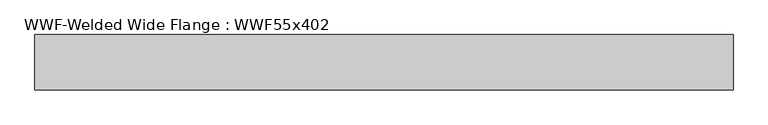
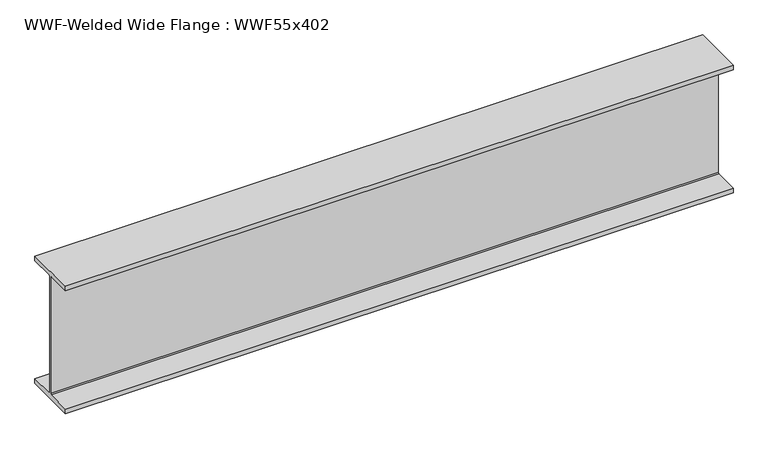
"""IFC4 building model written with IfcOpenShell, lengths in millimetres: beam geometry, WWF-Welded Wide Flange : WWF55x402."""

from ifc_helpers import new_model, si_unit, frame, origin, place, context, project, spatial, polyline, outline, extrude, source, transform, mapped, element, save


def wwf_welded_wide_flange_wwf55x402_e03ff242(model_context):
    return source(origin(), model_context, "Body", "SweptSolid", [
        extrude(outline(polyline([(274.955, -649.986), (274.955, -700.024), (-274.955, -700.024), (-274.955, -649.986), (-19.05, -649.986), (-8.001, -638.937), (-8.001, 638.937), (-19.05, 649.986), (-274.955, 649.986), (-274.955, 700.024), (274.955, 700.024), (274.955, 649.986), (19.05, 649.986), (8.001, 638.937), (8.001, -638.937), (19.05, -649.986), (274.955, -649.986)])), frame((-3472.2183929, 0.0, 0.0), z_axis=(1.0, 0.0, 0.0), x_axis=(0.0, 1.0, 0.0)), (0.0, 0.0, 1.0), 6944.4367858),
    ])


if __name__ == "__main__":
    model = new_model("IFC4")
    model_context = context("Model", 3, world=origin())
    ifc_project = project(units=[si_unit("LENGTHUNIT", "METRE", prefix="MILLI")], contexts=[model_context])
    site = spatial("IfcSite", under=ifc_project)
    building = spatial("IfcBuilding", under=site)
    placement = place(None, origin())
    wwf_welded_wide_flange_wwf55x402_shape = wwf_welded_wide_flange_wwf55x402_e03ff242(model_context)
    element("IfcBeam", 1, ObjectType="WWF-Welded Wide Flange : WWF55x402", at=placement, inside=building, context=model_context, shape_type="MappedRepresentation", body=[
        mapped(wwf_welded_wide_flange_wwf55x402_shape, transform((0.0, 0.0, 0.0), x_axis=(1.0, 0.0, 0.0), y_axis=(0.0, 1.0, 0.0), z_axis=(0.0, 0.0, 1.0))),
    ])
    save(model, "model.ifc")

# Revit data of these elements
# Type "WWF-Welded Wide Flange : WWF55x402"
#   Assembly Code = "B10"
#   Nominal d = "12"
#   W = 402
#   Length [instance default] = 1524 mm
#   bf = 549.91 mm
#   d = 1400.048 mm
#   k = 19.05 mm
#   tf = 50.038 mm
#   tw = 16.002 mm
#   A = 0.0761289 m²
#   Structural Material [instance default] = Steel ASTM A572
# Element 1 (IfcBeam, "WWF-Welded Wide Flange : WWF55x402")
#   Structural Material = Metal - Steel 43-275
#   Materials on its faces: "Metal - Steel 43-275"
# Materials
#   "Steel ASTM A572": class "Metal", colour RGB 247 247 247, transparency 0, Description = "Structural steel, high strength low alloy, ASTM - A572 - 50", Cost = 0
#   "Metal - Steel 43-275": class "Metal", colour RGB 247 247 247, transparency 0, Cost = 0
